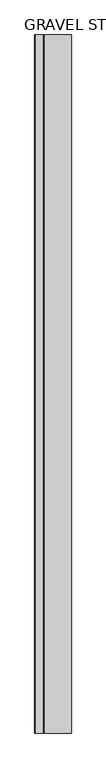
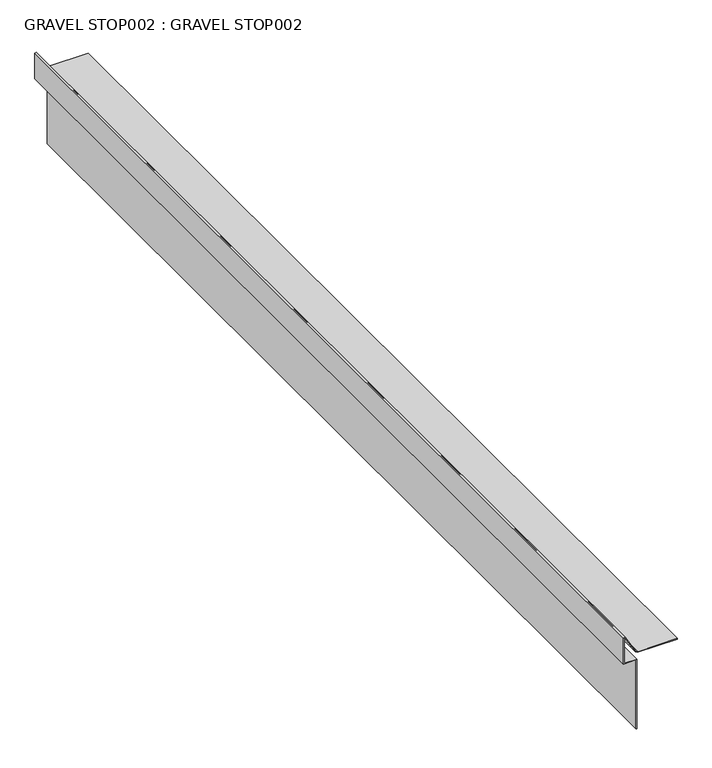
"""IFC4 building model written with IfcOpenShell, lengths in millimetres: proxy geometry, GRAVEL STOP002 : GRAVEL STOP002."""

from ifc_helpers import new_model, si_unit, frame, origin, place, context, project, spatial, polyline, outline, extrude, source, transform, mapped, element, save


def gravel_stop002_gravel_stop002_21b18a30(model_context):
    return source(origin(), model_context, "Body", "SweptSolid", [
        extrude(outline(polyline([(40295.3431515, -5034.9087762), (40294.5307525, -5037.9406906), (40240.9633674, -5037.9406906), (40240.9633674, -5013.600953), (40097.9858473, -5013.600953), (40097.9858473, -5012.189842), (40242.3744784, -5012.189842), (40242.3744784, -5036.5295796), (40293.447969, -5036.5295796), (40293.699878, -5035.5894424), (40258.5078708, -5015.2713276), (40255.9633674, -5010.8641185), (40255.9633674, -4933.0281058), (40257.3744784, -4933.0281058), (40257.3744784, -5010.4860124), (40259.5408757, -5014.2383227), (40295.3431515, -5034.9087762)])), frame((0.0, -1052.8906573, 0.0), z_axis=(0.0, 1.0, 0.0), x_axis=(0.0, 0.0, 1.0)), (0.0, 0.0, 1.0), 2000.25),
    ])


if __name__ == "__main__":
    model = new_model("IFC4")
    model_context = context("Model", 3, world=origin())
    ifc_project = project(units=[si_unit("LENGTHUNIT", "METRE", prefix="MILLI")], contexts=[model_context])
    site = spatial("IfcSite", under=ifc_project)
    building = spatial("IfcBuilding", under=site)
    placement = place(None, origin())
    gravel_stop002_gravel_stop002_shape = gravel_stop002_gravel_stop002_21b18a30(model_context)
    element("IfcBuildingElementProxy", 1, Name="GRAVEL STOP002 : GRAVEL STOP002", ObjectType="GRAVEL STOP002 : GRAVEL STOP002", at=placement, inside=building, context=model_context, shape_type="MappedRepresentation", body=[
        mapped(gravel_stop002_gravel_stop002_shape, transform((0.0, 0.0, 0.0), x_axis=(1.0, 0.0, 0.0), y_axis=(0.0, 1.0, 0.0), z_axis=(0.0, 0.0, 1.0))),
    ])
    save(model, "model.ifc")

# Revit data of these elements
# Type "GRAVEL STOP002 : GRAVEL STOP002"
#   NameOverride = "GRAVEL STOP002"
# Element 1 (IfcBuildingElementProxy, "GRAVEL STOP002 : GRAVEL STOP002")
#   Materials on its faces: "GRAVEL STOP REQUIRED WITH GRAVEL SURFACE SYSTEMS"
# Materials
#   "GRAVEL STOP REQUIRED WITH GRAVEL SURFACE SYSTEMS": class "Unassigned", colour RGB 170 170 127, transparency 0, Cost = 0
